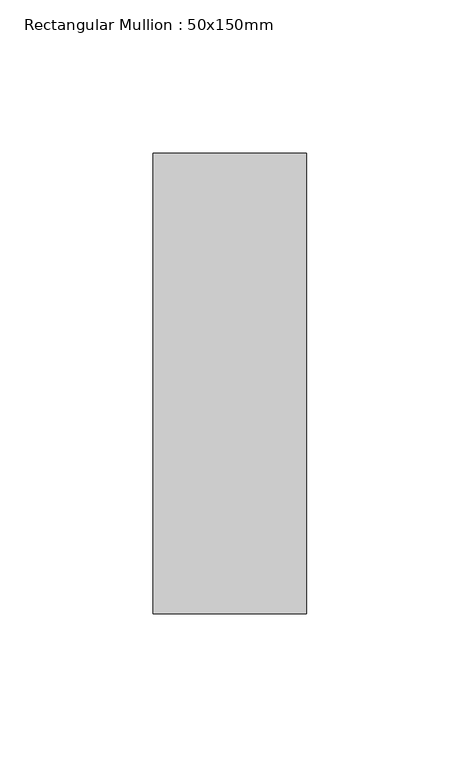
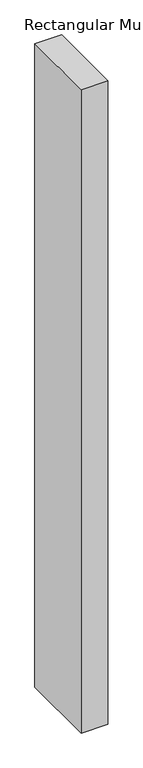
"""IFC4 building model written with IfcOpenShell, lengths in millimetres: member geometry, Rectangular Mullion : 50x150mm."""

from ifc_helpers import new_model, si_unit, frame, origin, place, context, project, spatial, polyline, outline, extrude, source, transform, mapped, element, save


def rectangular_mullion_50x150mm_7b764dd8(model_context):
    return source(origin(), model_context, "Body", "SweptSolid", [
        extrude(outline(polyline([(0.0, 75.0), (0.0, -75.0), (-50.0, -75.0), (-50.0, 75.0), (0.0, 75.0)])), frame((0.0, 0.0, -1275.0), z_axis=(0.0, 0.0, 1.0), x_axis=(1.0, 0.0, 0.0)), (0.0, 0.0, 1.0), 1275.0),
    ])


if __name__ == "__main__":
    model = new_model("IFC4")
    model_context = context("Model", 3, world=origin())
    ifc_project = project(units=[si_unit("LENGTHUNIT", "METRE", prefix="MILLI")], contexts=[model_context])
    site = spatial("IfcSite", under=ifc_project)
    building = spatial("IfcBuilding", under=site)
    placement = place(None, origin())
    rectangular_mullion_50x150mm_shape = rectangular_mullion_50x150mm_7b764dd8(model_context)
    element("IfcMember", 1, ObjectType="Rectangular Mullion : 50x150mm", at=placement, inside=building, context=model_context, shape_type="MappedRepresentation", body=[
        mapped(rectangular_mullion_50x150mm_shape, transform((0.0, 0.0, 0.0), x_axis=(1.0, 0.0, 0.0), y_axis=(0.0, 1.0, 0.0), z_axis=(0.0, 0.0, 1.0))),
    ])
    save(model, "model.ifc")

# Revit data of these elements
# Type "Rectangular Mullion : 50x150mm"
#   Keynote = "H11"
#   built-in parameter 1007304 = 0.492126 (stored number, unit not read)
#   built-in parameter 1007301 = 0.082021 (stored number, unit not read)
#   built-in parameter 1007300 = 0.082021 (stored number, unit not read)
# Element 1 (IfcMember, "Rectangular Mullion : 50x150mm")
#   Materials on its faces: "Aluminium"
# Materials
#   "Aluminium": class "Metal", colour RGB 247 247 247, transparency 0, Description = "Aluminium 6061", Cost = 0
